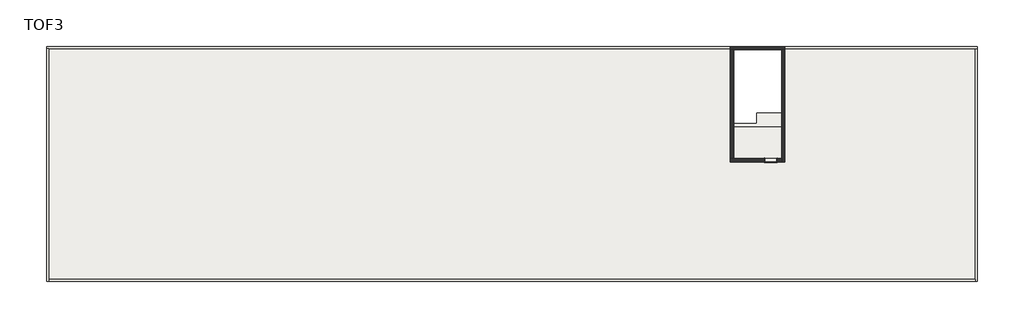
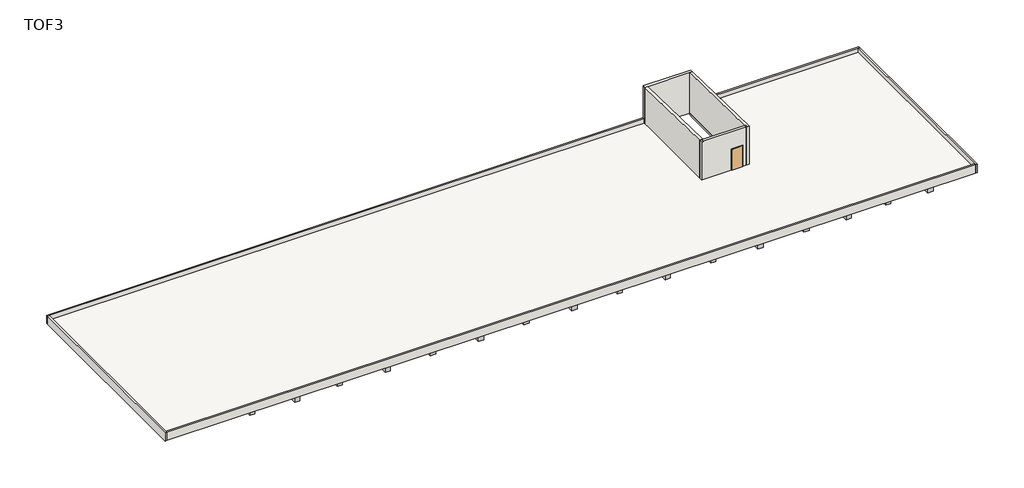
# One storey: 29 beams, 9 walls, 4 slabs, 1 door.
"""IFC4 building model written with IfcOpenShell, lengths in millimetres."""

import ifcopenshell
import ifcopenshell.guid

model = None  # the IFC model being written
_history = None  # IfcOwnerHistory: only IFC2X3 demands one
_inside = {}  # id of a spatial element -> (the spatial element, [elements in it])
_under = {}  # id of a project, library or spatial element -> (it, [spatial elements below it])
_declared = {}  # id of a project -> (the project, [libraries it declares])
_typed = {}  # id of a type object -> (the type object, [elements of that type])
_made_of = {}  # id of a material, layer set ... -> (it, [elements and type objects made of it])


def new_model(schema):
    """Start an empty IFC model of exactly this schema.

    Asked for "IFC4X3", IfcOpenShell would pick the latest addendum, in which some entities
    have other attributes; the version numbers below select the first issue.
    IFC2X3 requires an IfcOwnerHistory on every rooted entity: one is made here for all.
    """
    global model, _history
    if schema == "IFC4X3":
        model = ifcopenshell.file(schema_version=(4, 3, 0, 0))
    else:
        model = ifcopenshell.file(schema=schema)
    _inside.clear()
    _under.clear()
    _declared.clear()
    _typed.clear()
    _made_of.clear()
    _history = None
    if model.schema == "IFC2X3":
        org = make("IfcOrganization", Name="unknown")
        user = make(
            "IfcPersonAndOrganization",
            ThePerson=make("IfcPerson", FamilyName="unknown"),
            TheOrganization=org,
        )
        app = make(
            "IfcApplication",
            ApplicationDeveloper=org,
            Version="unknown",
            ApplicationFullName="unknown",
            ApplicationIdentifier="unknown",
        )
        _history = make(
            "IfcOwnerHistory",
            OwningUser=user,
            OwningApplication=app,
            ChangeAction="ADDED",
            CreationDate=0,
        )
    return model


def make(cls, **values):
    """One entity of the class cls with the attributes given. An attribute that is None is left unset."""
    return model.create_entity(
        cls, **{name: value for name, value in values.items() if value is not None}
    )


def rooted(cls, **values):
    """An entity with a GlobalId (a new one), such as an element, a storey or a relation."""
    return make(cls, GlobalId=ifcopenshell.guid.new(), OwnerHistory=_history, **values)


def si_unit(unit_type, name, prefix=None):
    """IfcSIUnit, for example si_unit("LENGTHUNIT", "METRE", prefix="MILLI")."""
    return make("IfcSIUnit", UnitType=unit_type, Prefix=prefix, Name=name)


def assignment(units):
    """IfcUnitAssignment: the units of a project."""
    return None if units is None else make("IfcUnitAssignment", Units=units)


def point(xyz):
    """IfcCartesianPoint."""
    return None if xyz is None else make("IfcCartesianPoint", Coordinates=xyz)


def direction(xyz):
    """IfcDirection."""
    return None if xyz is None else make("IfcDirection", DirectionRatios=xyz)


def frame(location, z_axis=None, x_axis=None):
    """IfcAxis2Placement3D, a coordinate frame: its origin and axes. An axis left out is left unset."""
    return make(
        "IfcAxis2Placement3D",
        Location=point(location),
        Axis=direction(z_axis),
        RefDirection=direction(x_axis),
    )


def origin():
    """The frame at (0, 0, 0) with its axes left unset."""
    return frame((0.0, 0.0, 0.0))


def origin_with_axes():
    """The frame at (0, 0, 0) with the z axis (0, 0, 1) and the x axis (1, 0, 0) written out."""
    return frame((0.0, 0.0, 0.0), z_axis=(0.0, 0.0, 1.0), x_axis=(1.0, 0.0, 0.0))


def place(relative_to, where):
    """IfcLocalPlacement: puts the frame where relative to a parent placement (None: the world)."""
    return make(
        "IfcLocalPlacement", PlacementRelTo=relative_to, RelativePlacement=where
    )


def context(
    kind, dimensions, precision=None, world=None, true_north=None, identifier=None
):
    """IfcGeometricRepresentationContext, for example the 3D "Model" context."""
    return make(
        "IfcGeometricRepresentationContext",
        ContextIdentifier=identifier,
        ContextType=kind,
        CoordinateSpaceDimension=dimensions,
        Precision=precision,
        WorldCoordinateSystem=world,
        TrueNorth=true_north,
    )


def project(units=None, contexts=None):
    """IfcProject with its units and contexts."""
    return rooted(
        "IfcProject",
        Name="project",
        RepresentationContexts=contexts,
        UnitsInContext=assignment(units),
    )


def spatial(cls, under=None, at=None, **own):
    """A site, building, storey or space (cls), placed at a placement, below another one or the project."""
    s = rooted(cls, ObjectPlacement=at, **own)
    if under is not None:
        _under.setdefault(under.id(), (under, []))[1].append(s)
    return s


def polyline(points):
    """IfcPolyline through the points."""
    return make("IfcPolyline", Points=[point(p) for p in points])


def outline(outer, holes=None, kind="AREA"):
    """IfcArbitraryClosedProfileDef: a profile drawn as a closed curve; with holes, ...WithVoids."""
    if holes is None:
        return make("IfcArbitraryClosedProfileDef", ProfileType=kind, OuterCurve=outer)
    return make(
        "IfcArbitraryProfileDefWithVoids",
        ProfileType=kind,
        OuterCurve=outer,
        InnerCurves=holes,
    )


def extrude(swept, where, along, depth):
    """IfcExtrudedAreaSolid: the profile swept, set in the frame where, extruded along a direction by depth."""
    return make(
        "IfcExtrudedAreaSolid",
        SweptArea=swept,
        Position=where,
        ExtrudedDirection=direction(along),
        Depth=depth,
    )


def faces_of(points, faces, orient=None, outer=None):
    """IfcFace entities. A face is a list of loops; a loop is a list of indices into points, from 0.

    orient and outer hold one flag for each loop. By default every Orientation is true, the
    first loop of a face is its IfcFaceOuterBound and the others are IfcFaceBound.
    """
    made = []
    for i, loops in enumerate(faces):
        bounds = []
        for j, loop in enumerate(loops):
            is_outer = j == 0 if outer is None else outer[i][j]
            bounds.append(
                make(
                    "IfcFaceOuterBound" if is_outer else "IfcFaceBound",
                    Bound=make("IfcPolyLoop", Polygon=[points[k] for k in loop]),
                    Orientation=True if orient is None else orient[i][j],
                )
            )
        made.append(make("IfcFace", Bounds=bounds))
    return made


def faceted_brep(points, faces, orient=None, outer=None, voids=None):
    """IfcFacetedBrep: a solid bounded by flat faces; with voids (closed shells), ...WithVoids."""
    shared = [point(p) for p in points]
    hull = make("IfcClosedShell", CfsFaces=faces_of(shared, faces, orient, outer))
    if voids is None:
        return make("IfcFacetedBrep", Outer=hull)
    return make(
        "IfcFacetedBrepWithVoids",
        Outer=hull,
        Voids=[
            make(cls, CfsFaces=faces_of(shared, fs, o, b)) for cls, fs, o, b in voids
        ],
    )


def shape(context_of_items, identifier, shape_type, items):
    """IfcShapeRepresentation: the items that make up one representation, for example the "Body"."""
    return make(
        "IfcShapeRepresentation",
        ContextOfItems=context_of_items,
        RepresentationIdentifier=identifier,
        RepresentationType=shape_type,
        Items=items,
    )


def source(mapping_origin, context_of_items, identifier, shape_type, items):
    """IfcRepresentationMap: a shape defined once, which mapped items show again and again."""
    return make(
        "IfcRepresentationMap",
        MappingOrigin=mapping_origin,
        MappedRepresentation=shape(context_of_items, identifier, shape_type, items),
    )


def transform(
    local_origin,
    x_axis=None,
    y_axis=None,
    z_axis=None,
    scale=None,
    scale2=None,
    scale3=None,
    uniform=True,
):
    """IfcCartesianTransformationOperator3D, or its non-uniform kind. x_axis, y_axis, z_axis: its Axis1, 2, 3."""
    if uniform:
        return make(
            "IfcCartesianTransformationOperator3D",
            Axis1=direction(x_axis),
            Axis2=direction(y_axis),
            LocalOrigin=point(local_origin),
            Scale=scale,
            Axis3=direction(z_axis),
        )
    return make(
        "IfcCartesianTransformationOperator3DnonUniform",
        Axis1=direction(x_axis),
        Axis2=direction(y_axis),
        LocalOrigin=point(local_origin),
        Scale=scale,
        Axis3=direction(z_axis),
        Scale2=scale2,
        Scale3=scale3,
    )


def mapped(mapping_source, mapping_target):
    """IfcMappedItem: shows the shape of a source again, moved by a transform."""
    return make(
        "IfcMappedItem", MappingSource=mapping_source, MappingTarget=mapping_target
    )


def made_of(thing, what):
    """Note that an element or type object is made of a material, layer set ...; save() writes the relation."""
    if what is not None:
        _made_of.setdefault(what.id(), (what, []))[1].append(thing)
    return thing


def element(
    cls,
    number,
    at=None,
    inside=None,
    cuts=None,
    type_object=None,
    material=None,
    context=None,
    identifier="Body",
    shape_type=None,
    held_by="IfcProductDefinitionShape",
    body=None,
    shapes=None,
    **own,
):
    """One element of the class cls, such as IfcWall. Its Tag is "e" and its number.

    at: its placement. inside: the storey or other place that contains it. cuts: it is an
    opening in that element (IfcRelVoidsElement). A single representation is given by context,
    identifier, shape_type and body (its items); several are given by shapes. held_by: the class
    of the entity that holds the representations. save() writes the other relations.
    """
    e = rooted(cls, Tag="e%d" % number, ObjectPlacement=at, **own)
    if body is not None:
        shapes = [shape(context, identifier, shape_type, body)]
    if shapes is not None:
        e.Representation = make(held_by, Representations=shapes)
    if inside is not None:
        _inside.setdefault(inside.id(), (inside, []))[1].append(e)
    if cuts is not None:
        rooted(
            "IfcRelVoidsElement", RelatingBuildingElement=cuts, RelatedOpeningElement=e
        )
    if type_object is not None:
        _typed.setdefault(type_object.id(), (type_object, []))[1].append(e)
    return made_of(e, material)


def aggregate(whole, parts):
    """IfcRelAggregates: a whole, such as a stair, and the parts it consists of."""
    return rooted("IfcRelAggregates", RelatingObject=whole, RelatedObjects=parts)


def save(model, path):
    """Write the relations noted so far, then the file.

    IfcRelAggregates (storeys below a building ...), IfcRelContainedInSpatialStructure (elements
    in a storey), IfcRelDefinesByType, IfcRelAssociatesMaterial and IfcRelDeclares: one each for
    every whole, place, type object, material and project.
    """
    for whole, parts in _under.values():
        aggregate(whole, parts)
    for where, things in _inside.values():
        rooted(
            "IfcRelContainedInSpatialStructure",
            RelatedElements=things,
            RelatingStructure=where,
        )
    for kind, things in _typed.values():
        rooted("IfcRelDefinesByType", RelatedObjects=things, RelatingType=kind)
    for what, things in _made_of.values():
        rooted("IfcRelAssociatesMaterial", RelatedObjects=things, RelatingMaterial=what)
    for by, libraries in _declared.values():
        rooted("IfcRelDeclares", RelatingContext=by, RelatedDefinitions=libraries)
    model.write(path)


def single_door_steel_e7c57604(model_context):
    return source(origin(), model_context, "Body", "SolidModel", [
        extrude(outline(polyline([(470.0, 155.0), (470.0, 120.0), (-470.0, 120.0), (-470.0, 155.0), (470.0, 155.0)])), origin_with_axes(), (0.0, 0.0, 1.0), 2250.0),
        faceted_brep([(470.0, 155.0, 0.0), (500.0, 155.0, 0.0), (500.0, -155.0, 0.0), (470.0, -155.0, 0.0), (470.0, -120.0, 0.0), (450.0, -120.0, 0.0), (450.0, 120.0, 0.0), (470.0, 120.0, 0.0), (470.0, 155.0, 2250.0), (-470.0, 155.0, 2250.0), (-470.0, 155.0, 0.0), (-500.0, 155.0, 0.0), (-500.0, 155.0, 2280.0), (500.0, 155.0, 2280.0), (500.0, -155.0, 2280.0), (-500.0, -155.0, 2280.0), (-500.0, -155.0, 0.0), (-470.0, -155.0, 0.0), (-470.0, -155.0, 2250.0), (470.0, -155.0, 2250.0), (470.0, -120.0, 2250.0), (-470.0, -120.0, 2250.0), (-470.0, -120.0, 0.0), (-450.0, -120.0, 0.0), (-450.0, -120.0, 2230.0), (450.0, -120.0, 2230.0), (450.0, 120.0, 2230.0), (-450.0, 120.0, 2230.0), (-450.0, 120.0, 0.0), (-470.0, 120.0, 0.0), (-470.0, 120.0, 2250.0), (470.0, 120.0, 2250.0)], [[[0, 1, 2, 3, 4, 5, 6, 7]], [[1, 0, 8, 9, 10, 11, 12, 13]], [[2, 1, 13, 14]], [[3, 2, 14, 15, 16, 17, 18, 19]], [[4, 3, 19, 20]], [[5, 4, 20, 21, 22, 23, 24, 25]], [[6, 5, 25, 26]], [[7, 6, 26, 27, 28, 29, 30, 31]], [[0, 7, 31, 8]], [[9, 30, 29, 10]], [[10, 29, 28, 23, 22, 17, 16, 11]], [[15, 12, 11, 16]], [[21, 18, 17, 22]], [[27, 24, 23, 28]], [[14, 13, 12, 15]], [[20, 19, 18, 21]], [[26, 25, 24, 27]], [[8, 31, 30, 9]]]),
    ])


model = new_model("IFC4")

# Units and contexts
model_context = context("Model", 3, world=origin())
ifc_project = project(units=[si_unit("LENGTHUNIT", "METRE", prefix="MILLI")], contexts=[model_context])

# Site, building, storey
site = spatial("IfcSite", under=ifc_project)
building = spatial("IfcBuilding", under=site)
storey = spatial("IfcBuildingStorey", under=building, Name="TOF3", Elevation=15409.9618634)

# Beams
placement = place(None, origin())
element("IfcBeam", 1, ObjectType="RC Beam_Rectangular : H_SB_AR_S16_AG_B450xH700_RG1", at=placement, inside=storey, context=model_context, shape_type="SweptSolid", body=[
    extrude(outline(polyline([(14775.0, 9849.5208589), (14775.0, 17199.5208589), (15225.0, 17199.5208589), (15225.0, 9849.5208589), (14775.0, 9849.5208589)])), frame((0.0, 0.0, 14709.9618634), z_axis=(0.0, 0.0, 1.0), x_axis=(1.0, 0.0, 0.0)), (0.0, 0.0, 1.0), 550.0),
])
element("IfcBeam", 2, ObjectType="RC Beam_Rectangular : H_SB_AR_S16_AG_B450xH700_RG1", at=placement, inside=storey, context=model_context, shape_type="SweptSolid", body=[
    extrude(outline(polyline([(22775.0, 9849.5208589), (22775.0, 17199.5208589), (23225.0, 17199.5208589), (23225.0, 9849.5208589), (22775.0, 9849.5208589)])), frame((0.0, 0.0, 14709.9618634), z_axis=(0.0, 0.0, 1.0), x_axis=(1.0, 0.0, 0.0)), (0.0, 0.0, 1.0), 550.0),
])
element("IfcBeam", 3, ObjectType="RC Beam_Rectangular : H_SB_AR_S16_AG_B450xH700_RG1", at=placement, inside=storey, context=model_context, shape_type="SweptSolid", body=[
    extrude(outline(polyline([(30775.0, 9849.5208589), (30775.0, 17199.5208589), (31225.0, 17199.5208589), (31225.0, 9849.5208589), (30775.0, 9849.5208589)])), frame((0.0, 0.0, 14709.9618634), z_axis=(0.0, 0.0, 1.0), x_axis=(1.0, 0.0, 0.0)), (0.0, 0.0, 1.0), 550.0),
])
element("IfcBeam", 4, ObjectType="RC Beam_Rectangular : H_SB_AR_S16_AG_B450xH700_RG1", at=placement, inside=storey, context=model_context, shape_type="SweptSolid", body=[
    extrude(outline(polyline([(38775.0, 9849.5208589), (38775.0, 17199.5208589), (39225.0, 17199.5208589), (39225.0, 9849.5208589), (38775.0, 9849.5208589)])), frame((0.0, 0.0, 14709.9618634), z_axis=(0.0, 0.0, 1.0), x_axis=(1.0, 0.0, 0.0)), (0.0, 0.0, 1.0), 550.0),
])
element("IfcBeam", 5, ObjectType="RC Beam_Rectangular : H_SB_AR_S16_AG_B450xH700_RB2", at=placement, inside=storey, context=model_context, shape_type="SweptSolid", body=[
    extrude(outline(polyline([(46775.0, 9849.5208589), (46775.0, 17199.5208589), (47225.0, 17199.5208589), (47225.0, 9849.5208589), (46775.0, 9849.5208589)])), frame((0.0, 0.0, 14709.9618634), z_axis=(0.0, 0.0, 1.0), x_axis=(1.0, 0.0, 0.0)), (0.0, 0.0, 1.0), 550.0),
])
element("IfcBeam", 6, ObjectType="RC Beam_Rectangular : H_SB_AR_S16_AG_B450xH700_RG1", at=placement, inside=storey, context=model_context, shape_type="SweptSolid", body=[
    extrude(outline(polyline([(61775.0, 9849.5208589), (61775.0, 17199.5208589), (62225.0, 17199.5208589), (62225.0, 9849.5208589), (61775.0, 9849.5208589)])), frame((0.0, 0.0, 14709.9618634), z_axis=(0.0, 0.0, 1.0), x_axis=(1.0, 0.0, 0.0)), (0.0, 0.0, 1.0), 550.0),
])
element("IfcBeam", 7, ObjectType="RC Beam_Rectangular : H_SB_AR_S16_AG_B450xH700_RG1", at=placement, inside=storey, context=model_context, shape_type="SweptSolid", body=[
    extrude(outline(polyline([(61775.0, 799.5208589), (61775.0, 9149.5208589), (62225.0, 9149.5208589), (62225.0, 799.5208589), (61775.0, 799.5208589)])), frame((0.0, 0.0, 14709.9618634), z_axis=(0.0, 0.0, 1.0), x_axis=(1.0, 0.0, 0.0)), (0.0, 0.0, 1.0), 550.0),
])
element("IfcBeam", 8, ObjectType="RC Beam_Rectangular : H_SB_AR_S16_AG_B450xH700_RG1", at=placement, inside=storey, context=model_context, shape_type="SweptSolid", body=[
    extrude(outline(polyline([(54775.0, 799.5208589), (54775.0, 9149.5208589), (55225.0, 9149.5208589), (55225.0, 799.5208589), (54775.0, 799.5208589)])), frame((0.0, 0.0, 14709.9618634), z_axis=(0.0, 0.0, 1.0), x_axis=(1.0, 0.0, 0.0)), (0.0, 0.0, 1.0), 550.0),
])
element("IfcBeam", 9, ObjectType="RC Beam_Rectangular : H_SB_AR_S16_AG_B450xH700_RG1", at=placement, inside=storey, context=model_context, shape_type="SweptSolid", body=[
    extrude(outline(polyline([(46775.0, 799.5208589), (46775.0, 9149.5208589), (47225.0, 9149.5208589), (47225.0, 799.5208589), (46775.0, 799.5208589)])), frame((0.0, 0.0, 14709.9618634), z_axis=(0.0, 0.0, 1.0), x_axis=(1.0, 0.0, 0.0)), (0.0, 0.0, 1.0), 550.0),
])
element("IfcBeam", 10, ObjectType="RC Beam_Rectangular : H_SB_AR_S16_AG_B450xH700_RG1", at=placement, inside=storey, context=model_context, shape_type="SweptSolid", body=[
    extrude(outline(polyline([(38775.0001504, 9149.7809743), (39224.9998496, 9149.2607435), (39215.3469712, 799.5208589), (38765.3466705, 799.5208589), (38775.0001504, 9149.7809743)])), frame((0.0, 0.0, 14709.9618634), z_axis=(0.0, 0.0, 1.0), x_axis=(1.0, 0.0, 0.0)), (0.0, 0.0, 1.0), 550.0),
])
element("IfcBeam", 11, ObjectType="RC Beam_Rectangular : H_SB_AR_S16_AG_B450xH700_RG1", at=placement, inside=storey, context=model_context, shape_type="SweptSolid", body=[
    extrude(outline(polyline([(30775.0, 799.5208589), (30775.0, 9149.5208589), (31225.0, 9149.5208589), (31225.0, 799.5208589), (30775.0, 799.5208589)])), frame((0.0, 0.0, 14709.9618634), z_axis=(0.0, 0.0, 1.0), x_axis=(1.0, 0.0, 0.0)), (0.0, 0.0, 1.0), 550.0),
])
element("IfcBeam", 12, ObjectType="RC Beam_Rectangular : H_SB_AR_S16_AG_B450xH700_RG1", at=placement, inside=storey, context=model_context, shape_type="SweptSolid", body=[
    extrude(outline(polyline([(22775.0, 799.5208589), (22775.0, 9149.5208589), (23225.0, 9149.5208589), (23225.0, 799.5208589), (22775.0, 799.5208589)])), frame((0.0, 0.0, 14709.9618634), z_axis=(0.0, 0.0, 1.0), x_axis=(1.0, 0.0, 0.0)), (0.0, 0.0, 1.0), 550.0),
])
element("IfcBeam", 13, ObjectType="RC Beam_Rectangular : H_SB_AR_S16_AG_B450xH700_RG1", at=placement, inside=storey, context=model_context, shape_type="SweptSolid", body=[
    extrude(outline(polyline([(14775.0, 799.5208589), (14775.0, 9149.5208589), (15225.0, 9149.5208589), (15225.0, 799.5208589), (14775.0, 799.5208589)])), frame((0.0, 0.0, 14709.9618634), z_axis=(0.0, 0.0, 1.0), x_axis=(1.0, 0.0, 0.0)), (0.0, 0.0, 1.0), 550.0),
])
element("IfcBeam", 14, ObjectType="RC Beam_Rectangular : H_SB_AR_S16_AG_B450xH700_RG1", at=placement, inside=storey, context=model_context, shape_type="SweptSolid", body=[
    extrude(outline(polyline([(7725.0, 799.5208589), (7275.0, 799.5208589), (7275.0, 9149.5208589), (7725.0, 9149.5208589), (7725.0, 799.5208589)])), frame((0.0, 0.0, 14709.9618634), z_axis=(0.0, 0.0, 1.0), x_axis=(1.0, 0.0, 0.0)), (0.0, 0.0, 1.0), 550.0),
])
element("IfcBeam", 15, ObjectType="RC Beam_Rectangular : H_SB_AR_S16_AG_B450xH700_RB1", at=placement, inside=storey, context=model_context, shape_type="SweptSolid", body=[
    extrude(outline(polyline([(11475.0, 9724.5208589), (11025.0, 9724.5208589), (11025.0, 17399.5208589), (11475.0, 17399.5208589), (11475.0, 9724.5208589)])), frame((0.0, 0.0, 14709.9618634), z_axis=(0.0, 0.0, 1.0), x_axis=(1.0, 0.0, 0.0)), (0.0, 0.0, 1.0), 550.0),
])
element("IfcBeam", 16, ObjectType="RC Beam_Rectangular : H_SB_AR_S16_AG_B450xH700_RB1A", at=placement, inside=storey, context=model_context, shape_type="SweptSolid", body=[
    extrude(outline(polyline([(11025.0, 9274.5208589), (11475.0, 9274.5208589), (11475.0, 599.5208589), (11025.0, 599.5208589), (11025.0, 9274.5208589)])), frame((0.0, 0.0, 14709.9618634), z_axis=(0.0, 0.0, 1.0), x_axis=(1.0, 0.0, 0.0)), (0.0, 0.0, 1.0), 550.0),
])
element("IfcBeam", 17, ObjectType="RC Beam_Rectangular : H_SB_AR_S16_AG_B450xH700_RB1", at=placement, inside=storey, context=model_context, shape_type="SweptSolid", body=[
    extrude(outline(polyline([(19225.0, 9724.5208589), (18775.0, 9724.5208589), (18775.0, 17399.5208589), (19225.0, 17399.5208589), (19225.0, 9724.5208589)])), frame((0.0, 0.0, 14709.9618634), z_axis=(0.0, 0.0, 1.0), x_axis=(1.0, 0.0, 0.0)), (0.0, 0.0, 1.0), 550.0),
])
element("IfcBeam", 18, ObjectType="RC Beam_Rectangular : H_SB_AR_S16_AG_B450xH700_RB1A", at=placement, inside=storey, context=model_context, shape_type="SweptSolid", body=[
    extrude(outline(polyline([(18775.0, 9274.5208589), (19225.0, 9274.5208589), (19225.0, 599.5208589), (18775.0, 599.5208589), (18775.0, 9274.5208589)])), frame((0.0, 0.0, 14709.9618634), z_axis=(0.0, 0.0, 1.0), x_axis=(1.0, 0.0, 0.0)), (0.0, 0.0, 1.0), 550.0),
])
element("IfcBeam", 19, ObjectType="RC Beam_Rectangular : H_SB_AR_S16_AG_B450xH700_RB1", at=placement, inside=storey, context=model_context, shape_type="SweptSolid", body=[
    extrude(outline(polyline([(27225.0, 9724.5208589), (26775.0, 9724.5208589), (26775.0, 17399.5208589), (27225.0, 17399.5208589), (27225.0, 9724.5208589)])), frame((0.0, 0.0, 14709.9618634), z_axis=(0.0, 0.0, 1.0), x_axis=(1.0, 0.0, 0.0)), (0.0, 0.0, 1.0), 550.0),
])
element("IfcBeam", 20, ObjectType="RC Beam_Rectangular : H_SB_AR_S16_AG_B450xH700_RB1A", at=placement, inside=storey, context=model_context, shape_type="SweptSolid", body=[
    extrude(outline(polyline([(26775.0, 9274.5208589), (27225.0, 9274.5208589), (27225.0, 599.5208589), (26775.0, 599.5208589), (26775.0, 9274.5208589)])), frame((0.0, 0.0, 14709.9618634), z_axis=(0.0, 0.0, 1.0), x_axis=(1.0, 0.0, 0.0)), (0.0, 0.0, 1.0), 550.0),
])
element("IfcBeam", 21, ObjectType="RC Beam_Rectangular : H_SB_AR_S16_AG_B450xH700_RB1", at=placement, inside=storey, context=model_context, shape_type="SweptSolid", body=[
    extrude(outline(polyline([(35225.0, 9724.5208589), (34775.0, 9724.5208589), (34775.0, 17399.5208589), (35225.0, 17399.5208589), (35225.0, 9724.5208589)])), frame((0.0, 0.0, 14709.9618634), z_axis=(0.0, 0.0, 1.0), x_axis=(1.0, 0.0, 0.0)), (0.0, 0.0, 1.0), 550.0),
])
element("IfcBeam", 22, ObjectType="RC Beam_Rectangular : H_SB_AR_S16_AG_B450xH700_RB1A", at=placement, inside=storey, context=model_context, shape_type="SweptSolid", body=[
    extrude(outline(polyline([(34775.0, 9274.5208589), (35225.0, 9274.5208589), (35225.0, 599.5208589), (34775.0, 599.5208589), (34775.0, 9274.5208589)])), frame((0.0, 0.0, 14709.9618634), z_axis=(0.0, 0.0, 1.0), x_axis=(1.0, 0.0, 0.0)), (0.0, 0.0, 1.0), 550.0),
])
element("IfcBeam", 23, ObjectType="RC Beam_Rectangular : H_SB_AR_S16_AG_B450xH700_RB1", at=placement, inside=storey, context=model_context, shape_type="SweptSolid", body=[
    extrude(outline(polyline([(43225.0, 9724.5208589), (42775.0, 9724.5208589), (42775.0, 17399.5208589), (43225.0, 17399.5208589), (43225.0, 9724.5208589)])), frame((0.0, 0.0, 14709.9618634), z_axis=(0.0, 0.0, 1.0), x_axis=(1.0, 0.0, 0.0)), (0.0, 0.0, 1.0), 550.0),
])
element("IfcBeam", 24, ObjectType="RC Beam_Rectangular : H_SB_AR_S16_AG_B450xH700_RB1A", at=placement, inside=storey, context=model_context, shape_type="SweptSolid", body=[
    extrude(outline(polyline([(42775.0, 9274.5208589), (43225.0, 9274.5208589), (43225.0, 599.5208589), (42775.0, 599.5208589), (42775.0, 9274.5208589)])), frame((0.0, 0.0, 14709.9618634), z_axis=(0.0, 0.0, 1.0), x_axis=(1.0, 0.0, 0.0)), (0.0, 0.0, 1.0), 550.0),
])
element("IfcBeam", 25, ObjectType="RC Beam_Rectangular : H_SB_AR_S16_AG_B450xH700_RB1A", at=placement, inside=storey, context=model_context, shape_type="SweptSolid", body=[
    extrude(outline(polyline([(50725.0, 599.5208589), (50725.0, 9224.5208589), (50825.0, 9224.5208589), (50825.0, 9149.5208589), (51175.0, 9149.5208589), (51175.0, 599.5208589), (50725.0, 599.5208589)])), frame((0.0, 0.0, 14709.9618634), z_axis=(0.0, 0.0, 1.0), x_axis=(1.0, 0.0, 0.0)), (0.0, 0.0, 1.0), 550.0),
])
element("IfcBeam", 26, ObjectType="RC Beam_Rectangular : H_SB_AR_S16_AG_B450xH700_RB1A", at=placement, inside=storey, context=model_context, shape_type="SweptSolid", body=[
    extrude(outline(polyline([(58725.0, 599.5208589), (58275.0, 599.5208589), (58275.0, 9149.5208589), (58725.0, 9149.5208589), (58725.0, 599.5208589)])), frame((0.0, 0.0, 14709.9618634), z_axis=(0.0, 0.0, 1.0), x_axis=(1.0, 0.0, 0.0)), (0.0, 0.0, 1.0), 550.0),
])
element("IfcBeam", 27, ObjectType="RC Beam_Rectangular : H_SB_AR_S16_AG_B450xH700_RB1A", at=placement, inside=storey, context=model_context, shape_type="SweptSolid", body=[
    extrude(outline(polyline([(65725.0, 599.5208589), (65275.0, 599.5208589), (65275.0, 9149.5208589), (65725.0, 9149.5208589), (65725.0, 599.5208589)])), frame((0.0, 0.0, 14709.9618634), z_axis=(0.0, 0.0, 1.0), x_axis=(1.0, 0.0, 0.0)), (0.0, 0.0, 1.0), 550.0),
])
element("IfcBeam", 28, ObjectType="RC Beam_Rectangular : H_SB_AR_S16_AG_B450xH700_RB1", at=placement, inside=storey, context=model_context, shape_type="SweptSolid", body=[
    extrude(outline(polyline([(58725.0, 9674.5208589), (58275.0, 9674.5208589), (58275.0, 17399.5208589), (58725.0, 17399.5208589), (58725.0, 9674.5208589)])), frame((0.0, 0.0, 14709.9618634), z_axis=(0.0, 0.0, 1.0), x_axis=(1.0, 0.0, 0.0)), (0.0, 0.0, 1.0), 550.0),
])
element("IfcBeam", 29, ObjectType="RC Beam_Rectangular : H_SB_AR_S16_AG_B450xH700_RB1", at=placement, inside=storey, context=model_context, shape_type="SweptSolid", body=[
    extrude(outline(polyline([(65725.0, 9674.5208589), (65275.0, 9674.5208589), (65275.0, 17399.5208589), (65725.0, 17399.5208589), (65725.0, 9674.5208589)])), frame((0.0, 0.0, 14709.9618634), z_axis=(0.0, 0.0, 1.0), x_axis=(1.0, 0.0, 0.0)), (0.0, 0.0, 1.0), 550.0),
])

# Door
single_door_steel_shape = single_door_steel_e7c57604(model_context)
element("IfcDoor", 30, ObjectType="Single Door_Steel : H_DR_AR_B12_Single Door_Steel_W1000xH2280_FSD2", at=placement, inside=storey, context=model_context, shape_type="MappedRepresentation", body=[
    mapped(single_door_steel_shape, transform((53850.0, 9274.5208589, 15409.9618634), x_axis=(-1.0, 0.0, 0.0), y_axis=(0.0, -1.0, 0.0), z_axis=(0.0, 0.0, 1.0))),
])

# Slabs
element("IfcSlab", 31, ObjectType="H_FL_AR_S17_RC Slab T150_RS1", at=placement, inside=storey, context=model_context, shape_type="Brep", body=[
    faceted_brep([(50825.0, 17549.5208589, 15259.9618634), (51075.0, 17549.5208589, 15259.9618634), (51075.0, 9399.5208589, 15259.9618634), (54650.0, 9399.5208589, 15259.9618634), (54650.0, 17114.5208589, 15259.9618634), (54650.0, 17549.5208589, 15259.9618634), (55350.0, 17549.5208589, 15259.9618634), (61700.0, 17549.5208589, 15259.9618634), (62300.0, 17549.5208589, 15259.9618634), (68700.0, 17549.5208589, 15259.9618634), (68900.0, 17549.5208589, 15259.9618634), (68900.0, 17199.5208589, 15259.9618634), (68900.0, 9849.5208589, 15259.9618634), (68900.0, 9799.5208589, 15259.9618634), (68900.0, 9199.5208589, 15259.9618634), (68900.0, 9149.5208589, 15259.9618634), (68900.0, 799.5208589, 15259.9618634), (68900.0, 449.5208589, 15259.9618634), (68700.0, 449.5208589, 15259.9618634), (62300.0, 449.5208589, 15259.9618634), (61700.0, 449.5208589, 15259.9618634), (55300.0, 449.5208589, 15259.9618634), (54700.0, 449.5208589, 15259.9618634), (50825.0, 449.5208589, 15259.9618634), (47300.0, 449.5208589, 15259.9618634), (46700.0, 449.5208589, 15259.9618634), (39300.0, 449.5208589, 15259.9618634), (38700.0, 449.5208589, 15259.9618634), (31300.0, 449.5208589, 15259.9618634), (30700.0, 449.5208589, 15259.9618634), (23300.0, 449.5208589, 15259.9618634), (22700.0, 449.5208589, 15259.9618634), (15300.0, 449.5208589, 15259.9618634), (14700.0, 449.5208589, 15259.9618634), (7800.0, 449.5208589, 15259.9618634), (7200.0, 449.5208589, 15259.9618634), (300.0, 449.5208589, 15259.9618634), (100.0, 449.5208589, 15259.9618634), (100.0, 799.5208589, 15259.9618634), (100.0, 9149.5208589, 15259.9618634), (100.0, 9849.5208589, 15259.9618634), (100.0, 17199.5208589, 15259.9618634), (100.0, 17549.5208589, 15259.9618634), (300.0, 17549.5208589, 15259.9618634), (7200.0, 17549.5208589, 15259.9618634), (7800.0, 17549.5208589, 15259.9618634), (14700.0, 17549.5208589, 15259.9618634), (15300.0, 17549.5208589, 15259.9618634), (22700.0, 17549.5208589, 15259.9618634), (23300.0, 17549.5208589, 15259.9618634), (30700.0, 17549.5208589, 15259.9618634), (31300.0, 17549.5208589, 15259.9618634), (38700.0, 17549.5208589, 15259.9618634), (39300.0, 17549.5208589, 15259.9618634), (46700.0, 17549.5208589, 15259.9618634), (47300.0, 17549.5208589, 15259.9618634), (50825.0, 17549.5208589, 15409.9618634), (100.0, 17549.5208589, 15409.9618634), (100.0, 17199.5208589, 15409.9618634), (100.0, 9849.5208589, 15409.9618634), (100.0, 9149.5208589, 15409.9618634), (100.0, 799.5208589, 15409.9618634), (100.0, 449.5208589, 15409.9618634), (50825.0, 449.5208589, 15409.9618634), (68900.0, 449.5208589, 15409.9618634), (68900.0, 799.5208589, 15409.9618634), (68900.0, 9149.5208589, 15409.9618634), (68900.0, 9199.5208589, 15409.9618634), (68900.0, 9799.5208589, 15409.9618634), (68900.0, 9849.5208589, 15409.9618634), (68900.0, 17199.5208589, 15409.9618634), (68900.0, 17549.5208589, 15409.9618634), (54650.0, 17549.5208589, 15409.9618634), (54650.0, 17399.5208589, 15409.9618634), (54650.0, 9674.5208589, 15409.9618634), (54650.0, 9399.5208589, 15409.9618634), (54647.235546, 9399.5208589, 15409.9618634), (51075.0, 9399.5208589, 15409.9618634), (51075.0, 17399.5208589, 15409.9618634), (51075.0, 17549.5208589, 15409.9618634)], [[[0, 1, 2, 3, 4, 5, 6, 7, 8, 9, 10, 11, 12, 13, 14, 15, 16, 17, 18, 19, 20, 21, 22, 23, 24, 25, 26, 27, 28, 29, 30, 31, 32, 33, 34, 35, 36, 37, 38, 39, 40, 41, 42, 43, 44, 45, 46, 47, 48, 49, 50, 51, 52, 53, 54, 55]], [[56, 57, 58, 59, 60, 61, 62, 63, 64, 65, 66, 67, 68, 69, 70, 71, 72, 73, 74, 75, 76, 77, 78, 79]], [[1, 0, 56, 79]], [[17, 16, 15, 14, 13, 12, 11, 10, 71, 70, 69, 68, 67, 66, 65, 64]], [[23, 22, 21, 20, 19, 18, 17, 64, 63]], [[37, 36, 35, 34, 33, 32, 31, 30, 29, 28, 27, 26, 25, 24, 23, 63, 62]], [[42, 41, 40, 39, 38, 37, 62, 61, 60, 59, 58, 57]], [[0, 55, 54, 53, 52, 51, 50, 49, 48, 47, 46, 45, 44, 43, 42, 57, 56]], [[2, 1, 79, 78, 77]], [[3, 2, 77, 76, 75]], [[5, 4, 3, 75, 74, 73, 72]], [[10, 9, 8, 7, 6, 5, 72, 71]]]),
])
element("IfcSlab", 32, ObjectType="H_FL_AR_S17_RC Slab T200_SS1", at=placement, inside=storey, context=model_context, shape_type="SweptSolid", body=[
    extrude(outline(polyline([(52810.0, 12829.5208589), (54650.0, 12829.5208589), (54650.0, 9399.5208589), (51075.0, 9399.5208589), (51075.0, 11579.5208589), (51075.0, 12029.5208589), (52810.0, 12029.5208589), (52810.0, 12829.5208589)])), frame((0.0, 0.0, 11209.9618634), z_axis=(0.0, 0.0, 1.0), x_axis=(1.0, 0.0, 0.0)), (0.0, 0.0, 1.0), 200.0),
])
element("IfcSlab", 33, ObjectType="H_FL_AR_S17_RC Slab T200_SS1", at=placement, inside=storey, context=model_context, shape_type="Brep", body=[
    faceted_brep([(51075.0, 11779.5208589, 15209.9618634), (54647.235546, 11779.5208589, 15209.9618634), (54647.235546, 9674.5208589, 15209.9618634), (54647.235546, 9399.5208589, 15209.9618634), (51075.0, 9399.5208589, 15209.9618634), (51075.0, 9674.5208589, 15209.9618634), (51075.0, 11779.5208589, 15409.9618634), (51075.0, 9399.5208589, 15409.9618634), (54647.235546, 9399.5208589, 15409.9618634), (54647.235546, 9674.5208589, 15409.9618634), (54647.235546, 11779.5208589, 15409.9618634)], [[[0, 1, 2, 3, 4, 5]], [[6, 7, 8, 9, 10]], [[1, 0, 6, 10]], [[3, 2, 1, 10, 9, 8]], [[4, 3, 8, 7]], [[0, 5, 4, 7, 6]]]),
])
element("IfcSlab", 34, ObjectType="H_RF_AR_B06_Roof Finish", at=placement, inside=storey, context=model_context, shape_type="Brep", body=[
    faceted_brep([(50825.0, 17649.5208589, 15409.9618634), (50825.0, 9399.5208589, 15409.9618634), (50825.0, 9149.5208589, 15409.9618634), (53350.0, 9149.5208589, 15409.9618634), (54350.0, 9149.5208589, 15409.9618634), (54650.0, 9149.5208589, 15409.9618634), (54907.0, 9149.5208589, 15409.9618634), (54907.0, 17649.5208589, 15409.9618634), (69150.0, 17649.5208589, 15409.9618634), (69150.0, 349.5208589, 15409.9618634), (-150.0, 349.5208589, 15409.9618634), (-150.0, 17649.5208589, 15409.9618634), (50825.0, 17649.5208589, 15759.9618634), (-150.0, 17649.5208589, 15759.9618634), (-150.0, 349.5208589, 15759.9618634), (69150.0, 349.5208589, 15759.9618634), (69150.0, 17649.5208589, 15759.9618634), (54907.0, 17649.5208589, 15759.9618634), (54907.0, 9149.5208589, 15759.9618634), (50825.0, 9149.5208589, 15759.9618634)], [[[0, 1, 2, 3, 4, 5, 6, 7, 8, 9, 10, 11]], [[12, 13, 14, 15, 16, 17, 18, 19]], [[2, 1, 0, 12, 19]], [[6, 5, 4, 3, 2, 19, 18]], [[7, 6, 18, 17]], [[8, 7, 17, 16]], [[9, 8, 16, 15]], [[10, 9, 15, 14]], [[11, 10, 14, 13]], [[0, 11, 13, 12]]]),
])

# Walls
element("IfcWall", 35, ObjectType="H_WA_AR_B02_Ext Wall_RC T250_W1_PH", at=placement, inside=storey, context=model_context, shape_type="Brep", body=[
    faceted_brep([(50825.0, 17549.5208589, 19049.9618634), (50825.0, 17549.5208589, 15409.9618634), (51075.0, 17549.5208589, 15409.9618634), (54650.0, 17549.5208589, 15409.9618634), (54900.0, 17549.5208589, 15409.9618634), (54900.0, 17549.5208589, 19049.9618634), (50825.0, 17799.5208589, 15409.9618634), (50825.0, 17799.5208589, 16149.9618634), (50825.0, 17799.5208589, 19049.9618634), (51075.0, 17799.5208589, 19049.9618634), (54650.0, 17799.5208589, 19049.9618634), (54900.0, 17799.5208589, 19049.9618634), (54900.0, 17799.5208589, 16149.9618634), (54900.0, 17799.5208589, 15409.9618634), (50825.0, 17649.5208589, 15409.9618634), (54900.0, 17649.5208589, 15409.9618634)], [[[0, 1, 2, 3, 4, 5]], [[6, 7, 8, 9, 10, 11, 12, 13]], [[4, 3, 2, 1, 14, 6, 13, 15]], [[0, 5, 11, 10, 9, 8]], [[4, 15, 13, 12, 11, 5]], [[0, 8, 7, 6, 14, 1]]]),
])
element("IfcWall", 36, ObjectType="H_WA_AR_B02_Ext Wall_RC T250_W1_PH", at=placement, inside=storey, context=model_context, shape_type="Brep", body=[
    faceted_brep([(54650.0, 9149.5208589, 15409.9618634), (54650.0, 9149.5208589, 18609.9618634), (54650.0, 9149.5208589, 19206.6647429), (54650.0, 9149.5208589, 19209.9618634), (54650.0, 9149.5208589, 19211.3736281), (54650.0, 9224.5208589, 19209.9618634), (54650.0, 9274.5208589, 19209.0206869), (54650.0, 17549.5208589, 19053.255981), (54650.0, 17549.5208589, 15409.9618634), (54650.0, 9399.5208589, 15409.9618634), (54900.0, 9149.5208589, 19211.3736281), (54900.0, 9149.5208589, 15409.9618634), (54900.0, 17549.5208589, 15409.9618634), (54900.0, 17549.5208589, 19049.9618634), (54900.0, 17549.5208589, 19053.255981), (54750.0, 9149.5208589, 19211.3736281)], [[[0, 1, 2, 3, 4, 5, 6, 7, 8, 9]], [[10, 11, 12, 13, 14]], [[0, 9, 8, 12, 11]], [[7, 6, 5, 4, 15, 10, 14]], [[7, 14, 13, 12, 8]], [[0, 11, 10, 15, 4, 3, 2, 1]]]),
])
element("IfcWall", 37, ObjectType="H_WA_AR_B02_Ext Wall_RC T250_W1_PH", at=placement, inside=storey, context=model_context, shape_type="Brep", body=[
    faceted_brep([(50975.0, 9399.5208589, 19209.9618634), (54750.0, 9399.5208589, 19209.9618634), (54750.0, 9399.5208589, 19206.6647429), (54650.0, 9399.5208589, 19206.6647429), (54650.0, 9399.5208589, 15409.9618634), (54350.0, 9399.5208589, 15409.9618634), (54350.0, 9399.5208589, 17689.9618634), (53350.0, 9399.5208589, 17689.9618634), (53350.0, 9399.5208589, 15409.9618634), (51075.0, 9399.5208589, 15409.9618634), (50825.0, 9399.5208589, 15409.9618634), (50825.0, 9399.5208589, 15759.9618634), (50825.0, 9399.5208589, 19206.6647429), (50975.0, 9399.5208589, 19206.6647429), (54750.0, 9149.5208589, 19209.9618634), (50975.0, 9149.5208589, 19209.9618634), (50975.0, 9149.5208589, 19206.6647429), (50825.0, 9149.5208589, 19206.6647429), (50825.0, 9149.5208589, 15759.9618634), (50825.0, 9149.5208589, 15409.9618634), (53350.0, 9149.5208589, 15409.9618634), (53350.0, 9149.5208589, 15759.9618634), (53350.0, 9149.5208589, 17689.9618634), (54350.0, 9149.5208589, 17689.9618634), (54350.0, 9149.5208589, 15759.9618634), (54350.0, 9149.5208589, 15409.9618634), (54650.0, 9149.5208589, 15409.9618634), (54650.0, 9149.5208589, 15759.9618634), (54650.0, 9149.5208589, 19206.6647429), (54750.0, 9149.5208589, 19206.6647429), (54750.0, 9299.5208589, 19209.9618634)], [[[0, 1, 2, 3, 4, 5, 6, 7, 8, 9, 10, 11, 12, 13]], [[14, 15, 16, 17, 18, 19, 20, 21, 22, 23, 24, 25, 26, 27, 28, 29]], [[5, 4, 26, 25]], [[10, 9, 8, 20, 19]], [[1, 0, 15, 14, 30]], [[7, 22, 21, 20, 8]], [[22, 7, 6, 23]], [[23, 6, 5, 25, 24]], [[29, 28, 3, 2]], [[4, 3, 28, 27, 26]], [[2, 1, 30, 14, 29]], [[13, 12, 17, 16]], [[10, 19, 18, 17, 12, 11]], [[0, 13, 16, 15]]]),
])
element("IfcWall", 38, ObjectType="H_WA_AR_B02_Ext Wall_RC T250_W1_PH", at=placement, inside=storey, context=model_context, shape_type="Brep", body=[
    faceted_brep([(51075.0, 9399.5208589, 19206.6677457), (51075.0, 9399.5208589, 15409.9618634), (51075.0, 17549.5208589, 15409.9618634), (51075.0, 17549.5208589, 19053.255981), (50825.0, 9399.5208589, 15409.9618634), (50825.0, 9399.5208589, 19206.6677457), (50825.0, 17549.5208589, 19053.255981), (50825.0, 17549.5208589, 19049.9618634), (50825.0, 17549.5208589, 15409.9618634)], [[[0, 1, 2, 3]], [[4, 5, 6, 7, 8]], [[2, 8, 7, 6, 3]], [[2, 1, 4, 8]], [[0, 3, 6, 5]], [[0, 5, 4, 1]]]),
])
element("IfcWall", 39, ObjectType="H_WA_AR_B02_Ext Wall_RC T150_parapet", at=placement, inside=storey, context=model_context, shape_type="Brep", body=[
    faceted_brep([(-300.0, 17649.5208589, 15409.9618634), (-150.0, 17649.5208589, 15409.9618634), (50825.0, 17649.5208589, 15409.9618634), (50825.0, 17649.5208589, 16149.9618634), (-150.0, 17649.5208589, 16149.9618634), (-300.0, 17649.5208589, 16149.9618634), (-300.0, 17799.5208589, 15409.9618634), (-300.0, 17799.5208589, 16149.9618634), (50825.0, 17799.5208589, 16149.9618634), (50825.0, 17799.5208589, 15409.9618634)], [[[0, 1, 2, 3, 4, 5]], [[6, 7, 8, 9]], [[2, 1, 0, 6, 9]], [[5, 4, 3, 8, 7]], [[0, 5, 7, 6]], [[3, 2, 9, 8]]]),
])
element("IfcWall", 40, ObjectType="H_WA_AR_B02_Ext Wall_RC T150_parapet", at=placement, inside=storey, context=model_context, shape_type="Brep", body=[
    faceted_brep([(69150.0, 17649.5208589, 15409.9618634), (69150.0, 349.5208589, 15409.9618634), (69150.0, 199.5208589, 15409.9618634), (69150.0, 199.5208589, 16149.9618634), (69150.0, 349.5208589, 16149.9618634), (69150.0, 17649.5208589, 16149.9618634), (69300.0, 17649.5208589, 15409.9618634), (69300.0, 17649.5208589, 16149.9618634), (69300.0, 199.5208589, 16149.9618634), (69300.0, 199.5208589, 15409.9618634)], [[[0, 1, 2, 3, 4, 5]], [[6, 7, 8, 9]], [[2, 1, 0, 6, 9]], [[5, 4, 3, 8, 7]], [[0, 5, 7, 6]], [[3, 2, 9, 8]]]),
])
element("IfcWall", 41, ObjectType="H_WA_AR_B02_Ext Wall_RC T150_parapet", at=placement, inside=storey, context=model_context, shape_type="SweptSolid", body=[
    extrude(outline(polyline([(-150.0, 349.5208589), (69150.0, 349.5208589), (69150.0, 199.5208589), (-150.0, 199.5208589), (-150.0, 349.5208589)])), frame((0.0, 0.0, 15409.9618634), z_axis=(0.0, 0.0, 1.0), x_axis=(1.0, 0.0, 0.0)), (0.0, 0.0, 1.0), 740.0),
])
element("IfcWall", 42, ObjectType="H_WA_AR_B02_Ext Wall_RC T150_parapet", at=placement, inside=storey, context=model_context, shape_type="Brep", body=[
    faceted_brep([(-300.0, 17649.5208589, 15409.9618634), (-300.0, 199.5208589, 15409.9618634), (-300.0, 199.5208589, 16149.9618634), (-300.0, 17649.5208589, 16149.9618634), (-150.0, 17649.5208589, 15409.9618634), (-150.0, 17649.5208589, 16149.9618634), (-150.0, 349.5208589, 16149.9618634), (-150.0, 199.5208589, 16149.9618634), (-150.0, 199.5208589, 15409.9618634), (-150.0, 349.5208589, 15409.9618634)], [[[0, 1, 2, 3]], [[4, 5, 6, 7, 8, 9]], [[1, 0, 4, 9, 8]], [[3, 2, 7, 6, 5]], [[0, 3, 5, 4]], [[2, 1, 8, 7]]]),
])
element("IfcWall", 43, ObjectType="H_WA_AR_B02_Ext Wall_RC T150_parapet", at=placement, inside=storey, context=model_context, shape_type="Brep", body=[
    faceted_brep([(54900.0, 17649.5208589, 15409.9618634), (54907.0, 17649.5208589, 15409.9618634), (69150.0, 17649.5208589, 15409.9618634), (69300.0, 17649.5208589, 15409.9618634), (69300.0, 17649.5208589, 16149.9618634), (69150.0, 17649.5208589, 16149.9618634), (54900.0, 17649.5208589, 16149.9618634), (54900.0, 17799.5208589, 15409.9618634), (54900.0, 17799.5208589, 16149.9618634), (69300.0, 17799.5208589, 16149.9618634), (69300.0, 17799.5208589, 15409.9618634)], [[[0, 1, 2, 3, 4, 5, 6]], [[7, 8, 9, 10]], [[3, 2, 1, 0, 7, 10]], [[6, 5, 4, 9, 8]], [[4, 3, 10, 9]], [[0, 6, 8, 7]]]),
])

save(model, "model.ifc")

# Revit data of these elements
# Type "RC Beam_Rectangular : H_SB_AR_S16_AG_B450xH700_RG1"
#   Type Comments = "AG"
#   Type Mark = "RG1"
#   H_Q'ty Cal Type Tag = "SB-Q1"
#   H_WM Code_1 = "A03AF032-00022 |  | M3 | Concrete Work | Superstructure Work | Structural Concrete | Cement Type-1 | 25MPa ≤ F'c (Cylinder Strength) < 30MPa |  |  |  |  | A03AF032-00022 Concrete Work Superstructure Work Structural Concrete  Cement Type-1 25MPa ≤ F'c (Cylinder Strength) < 30MPa      |  F'c (Cylinder Strength) = 24MPa"
#   H_WM Code_2 = "A03AD037-00002 |  | TON | Concrete Work | Substructure Work | Rebar Work | Deformed Bar (Non-Coat.) | 400MPa<Fy≤470MPa |  |  |  |  | A03AD037-00002 Concrete Work Substructure Work Rebar Work Deformed Bar (Non-Coat.)  400MPa<Fy≤470MPa      | ASTM A615 GRADE 60 (Fy=420MPa)"
#   H_WM Code_3 = "A03AF036-00001 |  | M2 | Concrete Work | Superstructure Work | Form Work (1 time in use) | Flat Form | Dressed Lumber, Plywood or Steel Form(Wood Planks are not Allowed) incl. Chamfer |  |  |  | A03AF036-00001 Concrete Work Superstructure Work Form Work (1 time in use) Flat Form     Dressed Lumber, Plywood or Steel Form(Wood Planks are not Allowed) incl. Chamfer   |"
#   중앙부 하부근 = ""
#   중앙부 상부근 = ""
#   중앙부 보조근 = ""
#   중앙부 늑근 = ""
#   외단부 하부근 = ""
#   외단부 상부근 = ""
#   외단부 보조근 = ""
#   외단부 늑근 = ""
#   부호 = "TG2"
#   내단부 하부근 = ""
#   내단부 상부근 = ""
#   내단부 보조근 = ""
#   내단부 늑근 = ""
#   ALL 하부근 = "3-D20"
#   ALL 상부근 = "4-D20"
#   ALL 보조근 = ""
#   ALL 늑근 = "2-D10 @120"
#   Width = 450 mm
#   Height = 700 mm
#   Length [instance default] = 1524 mm
#   b = 450 mm
#   h = 700 mm
#   hec_material3 [instance default] = none
#   hec_material2 [instance default] = none
#   hec_material1 [instance default] = none
#   Structural Material [instance default] = none
#   Assembly Code = ""
# Type "RC Beam_Rectangular : H_SB_AR_S16_AG_B450xH700_RB2"
#   Type Comments = "AG"
#   Type Mark = "RB2"
#   H_Q'ty Cal Type Tag = "SB-Q1"
#   H_WM Code_1 = "A03AF032-00022 |  | M3 | Concrete Work | Superstructure Work | Structural Concrete | Cement Type-1 | 25MPa ≤ F'c (Cylinder Strength) < 30MPa |  |  |  |  | A03AF032-00022 Concrete Work Superstructure Work Structural Concrete  Cement Type-1 25MPa ≤ F'c (Cylinder Strength) < 30MPa      |  F'c (Cylinder Strength) = 24MPa"
#   H_WM Code_2 = "A03AD037-00002 |  | TON | Concrete Work | Substructure Work | Rebar Work | Deformed Bar (Non-Coat.) | 400MPa<Fy≤470MPa |  |  |  |  | A03AD037-00002 Concrete Work Substructure Work Rebar Work Deformed Bar (Non-Coat.)  400MPa<Fy≤470MPa      | ASTM A615 GRADE 60 (Fy=420MPa)"
#   H_WM Code_3 = "A03AF036-00001 |  | M2 | Concrete Work | Superstructure Work | Form Work (1 time in use) | Flat Form | Dressed Lumber, Plywood or Steel Form(Wood Planks are not Allowed) incl. Chamfer |  |  |  | A03AF036-00001 Concrete Work Superstructure Work Form Work (1 time in use) Flat Form     Dressed Lumber, Plywood or Steel Form(Wood Planks are not Allowed) incl. Chamfer   |"
#   중앙부 하부근 = ""
#   중앙부 상부근 = ""
#   중앙부 보조근 = ""
#   중앙부 늑근 = ""
#   외단부 하부근 = ""
#   외단부 상부근 = ""
#   외단부 보조근 = ""
#   외단부 늑근 = ""
#   부호 = "TG2"
#   내단부 하부근 = ""
#   내단부 상부근 = ""
#   내단부 보조근 = ""
#   내단부 늑근 = ""
#   ALL 하부근 = "3-D20"
#   ALL 상부근 = "4-D20"
#   ALL 보조근 = ""
#   ALL 늑근 = "2-D10 @120"
#   Width = 450 mm
#   Height = 700 mm
#   Length [instance default] = 1524 mm
#   b = 450 mm
#   h = 700 mm
#   hec_material3 [instance default] = none
#   hec_material2 [instance default] = none
#   hec_material1 [instance default] = none
#   Structural Material [instance default] = none
#   Assembly Code = ""
# Type "RC Beam_Rectangular : H_SB_AR_S16_AG_B450xH700_RB1"
#   Type Comments = "AG"
#   Type Mark = "RB1"
#   H_Q'ty Cal Type Tag = "SB-Q1"
#   H_WM Code_1 = "A03AF032-00022 |  | M3 | Concrete Work | Superstructure Work | Structural Concrete | Cement Type-1 | 25MPa ≤ F'c (Cylinder Strength) < 30MPa |  |  |  |  | A03AF032-00022 Concrete Work Superstructure Work Structural Concrete  Cement Type-1 25MPa ≤ F'c (Cylinder Strength) < 30MPa      |  F'c (Cylinder Strength) = 24MPa"
#   H_WM Code_2 = "A03AD037-00002 |  | TON | Concrete Work | Substructure Work | Rebar Work | Deformed Bar (Non-Coat.) | 400MPa<Fy≤470MPa |  |  |  |  | A03AD037-00002 Concrete Work Substructure Work Rebar Work Deformed Bar (Non-Coat.)  400MPa<Fy≤470MPa      | ASTM A615 GRADE 60 (Fy=420MPa)"
#   H_WM Code_3 = "A03AF036-00001 |  | M2 | Concrete Work | Superstructure Work | Form Work (1 time in use) | Flat Form | Dressed Lumber, Plywood or Steel Form(Wood Planks are not Allowed) incl. Chamfer |  |  |  | A03AF036-00001 Concrete Work Superstructure Work Form Work (1 time in use) Flat Form     Dressed Lumber, Plywood or Steel Form(Wood Planks are not Allowed) incl. Chamfer   |"
#   중앙부 하부근 = ""
#   중앙부 상부근 = ""
#   중앙부 보조근 = ""
#   중앙부 늑근 = ""
#   외단부 하부근 = ""
#   외단부 상부근 = ""
#   외단부 보조근 = ""
#   외단부 늑근 = ""
#   부호 = "TG2"
#   내단부 하부근 = ""
#   내단부 상부근 = ""
#   내단부 보조근 = ""
#   내단부 늑근 = ""
#   ALL 하부근 = "3-D20"
#   ALL 상부근 = "4-D20"
#   ALL 보조근 = ""
#   ALL 늑근 = "2-D10 @120"
#   Width = 450 mm
#   Height = 700 mm
#   Length [instance default] = 1524 mm
#   b = 450 mm
#   h = 700 mm
#   hec_material3 [instance default] = none
#   hec_material2 [instance default] = none
#   hec_material1 [instance default] = none
#   Structural Material [instance default] = none
#   Assembly Code = ""
# Type "RC Beam_Rectangular : H_SB_AR_S16_AG_B450xH700_RB1A"
#   Type Comments = "AG"
#   Type Mark = "RB1A"
#   H_Q'ty Cal Type Tag = "SB-Q1"
#   H_WM Code_1 = "A03AF032-00022 |  | M3 | Concrete Work | Superstructure Work | Structural Concrete | Cement Type-1 | 25MPa ≤ F'c (Cylinder Strength) < 30MPa |  |  |  |  | A03AF032-00022 Concrete Work Superstructure Work Structural Concrete  Cement Type-1 25MPa ≤ F'c (Cylinder Strength) < 30MPa      |  F'c (Cylinder Strength) = 24MPa"
#   H_WM Code_2 = "A03AD037-00002 |  | TON | Concrete Work | Substructure Work | Rebar Work | Deformed Bar (Non-Coat.) | 400MPa<Fy≤470MPa |  |  |  |  | A03AD037-00002 Concrete Work Substructure Work Rebar Work Deformed Bar (Non-Coat.)  400MPa<Fy≤470MPa      | ASTM A615 GRADE 60 (Fy=420MPa)"
#   H_WM Code_3 = "A03AF036-00001 |  | M2 | Concrete Work | Superstructure Work | Form Work (1 time in use) | Flat Form | Dressed Lumber, Plywood or Steel Form(Wood Planks are not Allowed) incl. Chamfer |  |  |  | A03AF036-00001 Concrete Work Superstructure Work Form Work (1 time in use) Flat Form     Dressed Lumber, Plywood or Steel Form(Wood Planks are not Allowed) incl. Chamfer   |"
#   중앙부 하부근 = ""
#   중앙부 상부근 = ""
#   중앙부 보조근 = ""
#   중앙부 늑근 = ""
#   외단부 하부근 = ""
#   외단부 상부근 = ""
#   외단부 보조근 = ""
#   외단부 늑근 = ""
#   부호 = "TG2"
#   내단부 하부근 = ""
#   내단부 상부근 = ""
#   내단부 보조근 = ""
#   내단부 늑근 = ""
#   ALL 하부근 = "3-D20"
#   ALL 상부근 = "4-D20"
#   ALL 보조근 = ""
#   ALL 늑근 = "2-D10 @120"
#   Width = 450 mm
#   Height = 700 mm
#   Length [instance default] = 1524 mm
#   b = 450 mm
#   h = 700 mm
#   hec_material3 [instance default] = none
#   hec_material2 [instance default] = none
#   hec_material1 [instance default] = none
#   Structural Material [instance default] = none
#   Assembly Code = ""
# Type "Single Door_Steel : H_DR_AR_B12_Single Door_Steel_W1000xH2280_FSD2"
#   Type Mark = "440"
#   Analytic Construction = "<None>"
#   프레임 투영 외부. = 25 mm
#   프레임 투영 내부. = 25 mm
#   프레임 폭 = 75 mm
#   Height = 2280 mm
#   Width = 1000 mm
#   Define Thermal Properties by = 1
#   문 패널 = none
#   문 프레임 = none
#   Function = (empty or 0)
#   Wall Closure = (empty or 0)
# Type "H_FL_AR_S17_RC Slab T150_RS1"
#   Keynote = ""
#   Type Comments = "CV-AG"
#   Description = ""
#   Type Mark = "RS1"
#   H_Q'ty Cal Type Tag = "FL-Q1"
#   H_WM Code_1 = "A03AF032-00025 |  | M3 | Concrete Work | Superstructure Work | Structural Concrete | Cement Type-1 | 20MPa ≤ F'c (Cylinder Strength) < 25MPa |  |  |  |  | A03AF032-00025 Concrete Work Superstructure Work Structural Concrete  Cement Type-1 20MPa ≤ F'c (Cylinder Strength) < 25MPa      |  F'c (Cylinder Strength) = 24MPa"
#   H_WM Code_2 = "A03AF037-00003 |  | TON | Concrete Work | Superstructure Work | Rebar Work | Deformed Bar (Non-Coat.) | 300MPa<Fy≤400MPa |  |  |  |  | A03AF037-00003 Concrete Work Superstructure Work Rebar Work Deformed Bar (Non-Coat.)  300MPa<Fy≤400MPa      | ASTM A615 GRADE 60 (Fy=420MPa)"
#   H_WM Code_3 = "A03AF036-00001 |  | M2 | Concrete Work | Superstructure Work | Form Work (1 time in use) | Flat Form | Dressed Lumber, Plywood or Steel Form(Wood Planks are not Allowed) incl. Chamfer |  |  |  | A03AF036-00001 Concrete Work Superstructure Work Form Work (1 time in use) Flat Form     Dressed Lumber, Plywood or Steel Form(Wood Planks are not Allowed) incl. Chamfer   |"
#   H_WM Code_4 = "A04AQ089-00001 |  | M3 | Finishing Work | Roof Work | Protective Concrete w/ Steel Trowel Finish |  |  |  | A04AQ089-00001 Finishing Work Roof Work Protective Concrete w/ Steel Trowel Finish         | Protective Concrete w/ Steel Trowel Finish (Slope 1%)"
#   H_WM Code_5 = "A04AQ088-00004 |  | M2 | Finishing Work | Roof Work | Roof Insulation | Rigid Extruded Polystyrene Foam Insulation |  | 100mm≤THK | THK=(  )mm |  | A04AQ088-00004 Finishing Work Roof Work Roof Insulation Rigid Extruded Polystyrene Foam Insulation       100mm≤THK | XPS\nTHK=( 220 )mm"
#   H_WM Code_6 = "A04AQ310-00001 |  | M2 | Finishing Work | Roof Work | Waterproofing Membrane | EPDM(or Equivalent) | w/ Accessories | THK=(  )mm |  | A04AQ310-00001 Finishing Work Roof Work Waterproofing Membrane EPDM(or Equivalent)     w/ Accessories   | Mesh Size=DIA( #8 )mm x ( 150 )mm x (150  )mm"
#   H_WM Code_7 = "A04AQ089-00001 |  | M3 | Finishing Work | Roof Work | Protective Concrete w/ Steel Trowel Finish |  |  |  | A04AQ089-00001 Finishing Work Roof Work Protective Concrete w/ Steel Trowel Finish         | Protective Concrete w/ Steel Trowel Finish"
#   H_Rebar ratio = 0.1
#   Function = 1
#   Layers, outside or top first: 150 mm "00_Concrete_Reinf. Conc." (function 1)
# Type "H_FL_AR_S17_RC Slab T200_SS1"
#   Keynote = ""
#   Type Comments = "CV-AG"
#   Description = ""
#   Type Mark = "SS1"
#   H_Q'ty Cal Type Tag = "RF-Q1"
#   H_WM Code_1 = "A04AQ310-00001 |  | M2 | Finishing Work | Roof Work | Waterproofing Membrane | EPDM(or Equivalent) | w/ Accessories | THK=(  )mm |  | A04AQ310-00001 Finishing Work Roof Work Waterproofing Membrane EPDM(or Equivalent)     w/ Accessories   | EPDM(or Equivalent)\nTHK=( 4 )mm"
#   H_WM Code_2 = "A04AQ088-00002 |  | M2 | Finishing Work | Roof Work | Roof Insulation | Rigid Extruded Polystyrene Foam Insulation |  | 50mm≤THK<75mm | THK=(  )mm |  | A04AQ088-00002 Finishing Work Roof Work Roof Insulation Rigid Extruded Polystyrene Foam Insulation       50mm≤THK<75mm | XPS\nTHK=( 120 )mm"
#   H_WM Code_3 = "A04AQ012-00001 |  | M2 | Finishing Work | Roof Work | PE Sheet (Vapor Barrier) |  | THK=(  )mm |  | A04AQ012-00001 Finishing Work Roof Work PE Sheet (Vapor Barrier)         | Mesh Size=DIA( #8 )mm x ( 150 )mm x (150  )mm"
#   H_WM Code_4 = "A04AQ089-00001 |  | M3 | Finishing Work | Roof Work | Protective Concrete w/ Steel Trowel Finish |  |  |  | A04AQ089-00001 Finishing Work Roof Work Protective Concrete w/ Steel Trowel Finish         | Protective Concrete w/ Steel Trowel Finish (Slope 1%)"
#   H_Rebar ratio = 0.1
#   Function = 1
#   Layers, outside or top first: 200 mm "00_Concrete_Reinf. Conc." (function 1)
# Type "H_RF_AR_B06_Roof Finish"
#   Keynote = ""
#   Type Comments = ""
#   Description = ""
#   H_Q'ty Cal Type Tag = "WA-Q1"
#   H_WM Code_1 = "A03AF032-00022 |  | M3 | Concrete Work | Superstructure Work | Structural Concrete | Cement Type-1 | 25MPa ≤ F'c (Cylinder Strength) < 30MPa |  |  |  |  | A03AF032-00022 Concrete Work Superstructure Work Structural Concrete  Cement Type-1 25MPa ≤ F'c (Cylinder Strength) < 30MPa      |"
#   H_WM Code_2 = "A03AD037-00002 |  | TON | Concrete Work | Substructure Work | Rebar Work | Deformed Bar (Non-Coat.) | 400MPa<Fy≤470MPa |  |  |  |  | A03AD037-00002 Concrete Work Substructure Work Rebar Work Deformed Bar (Non-Coat.)  400MPa<Fy≤470MPa      |"
#   H_WM Code_3 = "A03AD035-00001 |  | M2 | Concrete Work | Substructure Work | Form Work (3 times in use) | Flat Form | Dressed Lumber, Plywood or Steel Form(Wood Planks are not Allowed) incl. Chamfer |  |  |  | A03AD035-00001 Concrete Work Substructure Work Form Work (3 times in use) Flat Form     Dressed Lumber, Plywood or Steel Form(Wood Planks are not Allowed) incl. Chamfer   |"
#   H_WM Code_4 = "A03AH056-00001 |  | M2 | Concrete Work | Concrete Protective Coating (U/G) | Bitumen/Bituminous/Asphalt Coating |  |  | A03AH056-00001 Concrete Work Concrete Protective Coating (U/G) Bitumen/Bituminous/Asphalt Coating         | Exterior Protection"
#   H_WM Code_5 = "A03AD047-00004 |  | M2 | Concrete Work | Substructure Work | Insulation under Ground Floor | Extruded Polystyrene Insulation Board |  | 100mm≤THK | THK=(  )mm |  | A03AD047-00004 Concrete Work Substructure Work Insulation under Ground Floor Extruded Polystyrene Insulation Board       100mm≤THK | Interior Paint"
#   Function = 1
#   Layers, outside or top first: 350 mm "Roofs" (function 4)
# Type "H_WA_AR_B02_Ext Wall_RC T250_W1_PH"
#   Type Comments = "CV-AG"
#   Type Mark = "W1"
#   H_Q'ty Cal Type Tag = "WA-Q1"
#   H_WM Code_1 = "A03AD032-00025 |  | M3 | Concrete Work | Substructure Work | Structural Concrete | Cement Type-1 | 20MPa ≤ F'c (Cylinder Strength) < 25MPa |  |  |  |  | A03AD032-00025 Concrete Work Substructure Work Structural Concrete  Cement Type-1 20MPa ≤ F'c (Cylinder Strength) < 25MPa      | ASTM C150 Type I or Type IA \nF'c (Cylinder Strength) = 24MPa"
#   H_WM Code_2 = "A03AD037-00002 |  | TON | Concrete Work | Substructure Work | Rebar Work | Deformed Bar (Non-Coat.) | 400MPa<Fy≤470MPa |  |  |  |  | A03AD037-00002 Concrete Work Substructure Work Rebar Work Deformed Bar (Non-Coat.)  400MPa<Fy≤470MPa      | ASTM A615 GRADE 60 (Fy=420MPa)"
#   H_WM Code_3 = "A03AD036-00001 |  | M2 | Concrete Work | Substructure Work | Form Work (1 time in use) | Flat Form | Dressed Lumber, Plywood or Steel Form(Wood Planks are not Allowed) incl. Chamfer |  |  |  | A03AD036-00001 Concrete Work Substructure Work Form Work (1 time in use) Flat Form     Dressed Lumber, Plywood or Steel Form(Wood Planks are not Allowed) incl. Chamfer   |"
#   H_Rebar ratio = 0.12
#   Layers, outside or top first: 250 mm "00_Concrete_Reinf. Conc." (function 1)
# Type "H_WA_AR_B02_Ext Wall_RC T150_parapet"
#   Type Comments = "CV-AG"
#   Type Mark = "parapet"
#   H_Q'ty Cal Type Tag = "WA-Q1"
#   H_WM Code_1 = "A04AS178-00001 |  | M2 | Finishing Work | Exterior/Interior Finish Work | Gypsumboard Partition Wall (Removable Type) | Fire Protective Rating: N/A, 1-Layer Gypsum Board to Both Sides | Mineral Wool (Rock Wool) | Including Supporting Frame(Stud) & Accessories | 1-Layer Gypsumboard THK=9.5mm | Insulation THK=(  )mm |  | A04AS178-00001 Finishing Work Exterior/Interior Finish Work Gypsumboard Partition Wall (Removable Type) Fire Protective Rating: N/A, 1-Layer Gypsum Board to Both Sides   Mineral Wool (Rock Wool)  Including Supporting Frame(Stud) & Accessories  1-Layer Gypsumboard THK=9.5mm | Glass wall (WM 없음)"
#   H_WM Code_2 = "A03AD037-00002 |  | TON | Concrete Work | Substructure Work | Rebar Work | Deformed Bar (Non-Coat.) | 400MPa<Fy≤470MPa |  |  |  |  | A03AD037-00002 Concrete Work Substructure Work Rebar Work Deformed Bar (Non-Coat.)  400MPa<Fy≤470MPa      | ASTM A615 GRADE 60 (Fy=420MPa)"
